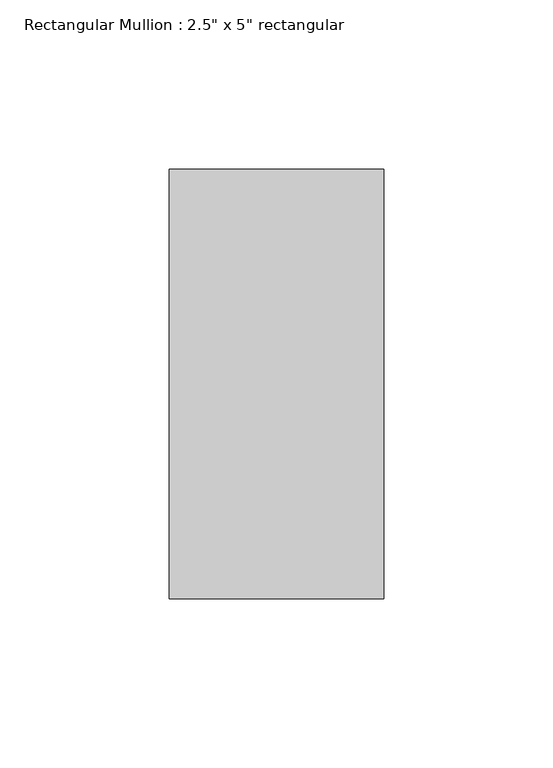
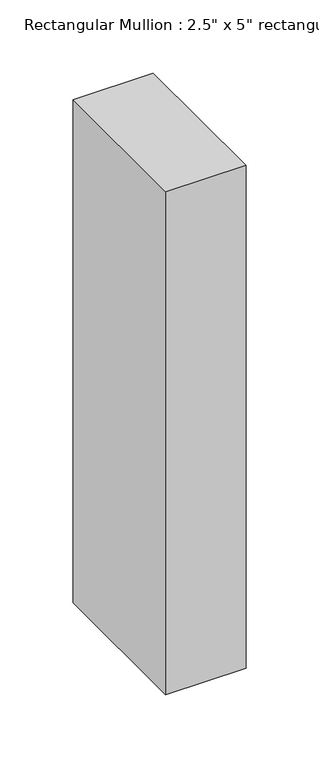
"""IFC4 building model written with IfcOpenShell, lengths in millimetres: member geometry."""

from ifc_helpers import new_model, si_unit, frame, origin, place, context, project, spatial, polyline, outline, extrude, source, transform, mapped, element, save


def member_0385dd90(model_context):
    return source(origin(), model_context, "Body", "SweptSolid", [
        extrude(outline(polyline([(31.75, 63.5), (31.75, -63.5), (-31.75, -63.5), (-31.75, 63.5), (31.75, 63.5)])), frame((0.0, 0.0, -420.214047), z_axis=(0.0, 0.0, 1.0), x_axis=(1.0, 0.0, 0.0)), (0.0, 0.0, 1.0), 420.214047),
    ])


if __name__ == "__main__":
    model = new_model("IFC4")
    model_context = context("Model", 3, world=origin())
    ifc_project = project(units=[si_unit("LENGTHUNIT", "METRE", prefix="MILLI")], contexts=[model_context])
    site = spatial("IfcSite", under=ifc_project)
    building = spatial("IfcBuilding", under=site)
    placement = place(None, origin())
    member_shape = member_0385dd90(model_context)
    element("IfcMember", 1, ObjectType="Rectangular Mullion : 2.5\" x 5\" rectangular", at=placement, inside=building, context=model_context, shape_type="MappedRepresentation", body=[
        mapped(member_shape, transform((0.0, 0.0, 0.0), x_axis=(1.0, 0.0, 0.0), y_axis=(0.0, 1.0, 0.0), z_axis=(0.0, 0.0, 1.0))),
    ])
    save(model, "model.ifc")

# Revit data of these elements
# Type "Rectangular Mullion : 2.5\" x 5\" rectangular"
#   built-in parameter 1007304 = 0.416667 (stored number, unit not read)
#   built-in parameter 1007301 = 0.104167 (stored number, unit not read)
#   built-in parameter 1007300 = 0.104167 (stored number, unit not read)
# Element 1 (IfcMember, "Rectangular Mullion : 2.5\" x 5\" rectangular")
#   Materials on its faces: "Metal - Aluminum 2"
# Materials
#   "Metal - Aluminum 2": class "Metal", colour RGB 189 187 185, transparency 0
